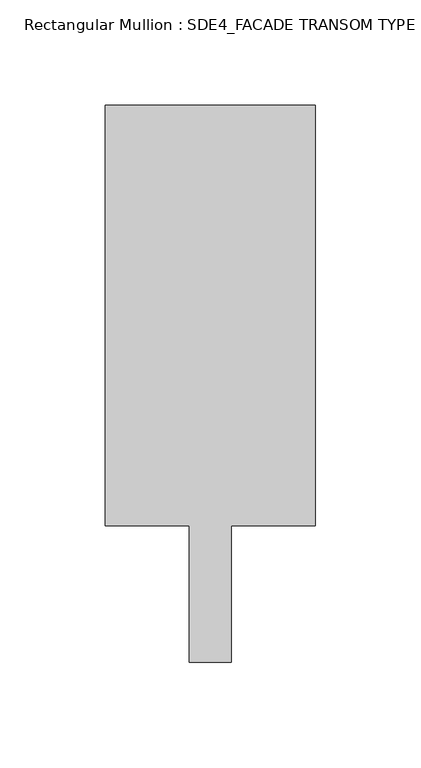
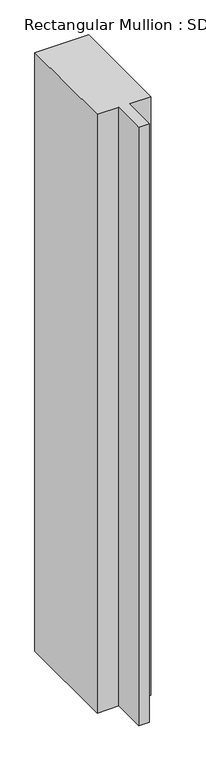
"""IFC4 building model written with IfcOpenShell, lengths in millimetres: member geometry, Rectangular Mullion : SDE4_FACADE TRANSOM TYPE 2."""

from ifc_helpers import new_model, si_unit, frame, origin, place, context, project, spatial, polyline, outline, extrude, source, transform, mapped, element, save


def rectangular_mullion_sde4_facade_transom_type_2_2d87ed10(model_context):
    return source(origin(), model_context, "Body", "SweptSolid", [
        extrude(outline(polyline([(50.0, 132.5), (50.0, -67.5), (10.0, -67.5), (10.0, -132.5), (-10.0, -132.5), (-10.0, -67.5), (-50.0, -67.5), (-50.0, 132.5), (50.0, 132.5)])), frame((0.0, 0.0, -1176.8857869), z_axis=(0.0, 0.0, 1.0), x_axis=(1.0, 0.0, 0.0)), (0.0, 0.0, 1.0), 1176.8857869),
    ])


if __name__ == "__main__":
    model = new_model("IFC4")
    model_context = context("Model", 3, world=origin())
    ifc_project = project(units=[si_unit("LENGTHUNIT", "METRE", prefix="MILLI")], contexts=[model_context])
    site = spatial("IfcSite", under=ifc_project)
    building = spatial("IfcBuilding", under=site)
    placement = place(None, origin())
    rectangular_mullion_sde4_facade_transom_type_2_shape = rectangular_mullion_sde4_facade_transom_type_2_2d87ed10(model_context)
    element("IfcMember", 1, ObjectType="Rectangular Mullion : SDE4_FACADE TRANSOM TYPE 2", at=placement, inside=building, context=model_context, shape_type="MappedRepresentation", body=[
        mapped(rectangular_mullion_sde4_facade_transom_type_2_shape, transform((0.0, 0.0, 0.0), x_axis=(1.0, 0.0, 0.0), y_axis=(0.0, 1.0, 0.0), z_axis=(0.0, 0.0, 1.0))),
    ])
    save(model, "model.ifc")

# Revit data of these elements
# Type "Rectangular Mullion : SDE4_FACADE TRANSOM TYPE 2"
#   built-in parameter 1007322 = 0.869423 (stored number, unit not read)
#   built-in parameter 1007321 = 0.164042 (stored number, unit not read)
#   built-in parameter 1007320 = 0.164042 (stored number, unit not read)
